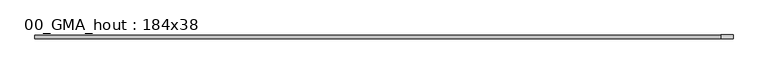
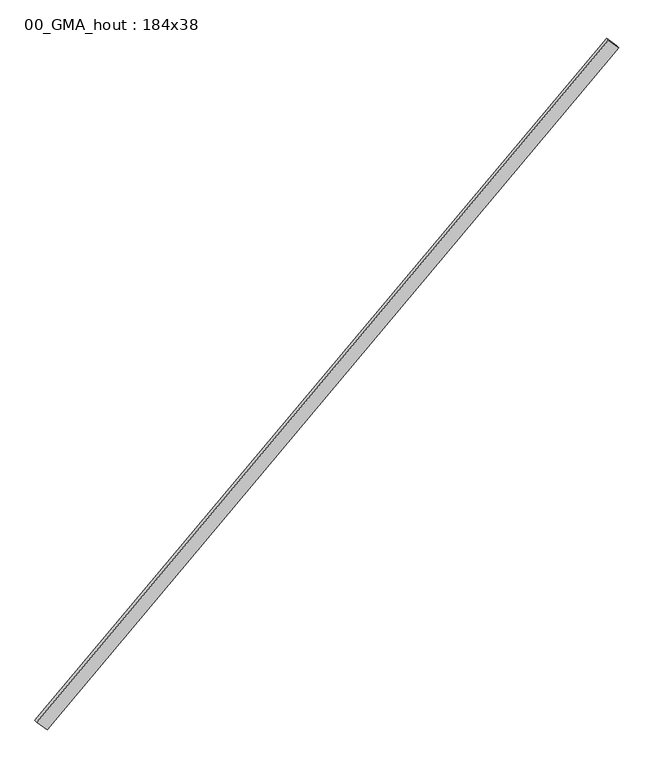
"""IFC4 building model written with IfcOpenShell, lengths in millimetres: proxy geometry, 00_GMA_hout : 184x38."""

import ifcopenshell
import ifcopenshell.guid

model = None  # the IFC model being written
_history = None  # IfcOwnerHistory: only IFC2X3 demands one
_inside = {}  # id of a spatial element -> (the spatial element, [elements in it])
_under = {}  # id of a project, library or spatial element -> (it, [spatial elements below it])
_declared = {}  # id of a project -> (the project, [libraries it declares])
_typed = {}  # id of a type object -> (the type object, [elements of that type])
_made_of = {}  # id of a material, layer set ... -> (it, [elements and type objects made of it])


def new_model(schema):
    """Start an empty IFC model of exactly this schema.

    Asked for "IFC4X3", IfcOpenShell would pick the latest addendum, in which some entities
    have other attributes; the version numbers below select the first issue.
    IFC2X3 requires an IfcOwnerHistory on every rooted entity: one is made here for all.
    """
    global model, _history
    if schema == "IFC4X3":
        model = ifcopenshell.file(schema_version=(4, 3, 0, 0))
    else:
        model = ifcopenshell.file(schema=schema)
    _inside.clear()
    _under.clear()
    _declared.clear()
    _typed.clear()
    _made_of.clear()
    _history = None
    if model.schema == "IFC2X3":
        org = make("IfcOrganization", Name="unknown")
        user = make(
            "IfcPersonAndOrganization",
            ThePerson=make("IfcPerson", FamilyName="unknown"),
            TheOrganization=org,
        )
        app = make(
            "IfcApplication",
            ApplicationDeveloper=org,
            Version="unknown",
            ApplicationFullName="unknown",
            ApplicationIdentifier="unknown",
        )
        _history = make(
            "IfcOwnerHistory",
            OwningUser=user,
            OwningApplication=app,
            ChangeAction="ADDED",
            CreationDate=0,
        )
    return model


def make(cls, **values):
    """One entity of the class cls with the attributes given. An attribute that is None is left unset."""
    return model.create_entity(
        cls, **{name: value for name, value in values.items() if value is not None}
    )


def rooted(cls, **values):
    """An entity with a GlobalId (a new one), such as an element, a storey or a relation."""
    return make(cls, GlobalId=ifcopenshell.guid.new(), OwnerHistory=_history, **values)


def si_unit(unit_type, name, prefix=None):
    """IfcSIUnit, for example si_unit("LENGTHUNIT", "METRE", prefix="MILLI")."""
    return make("IfcSIUnit", UnitType=unit_type, Prefix=prefix, Name=name)


def assignment(units):
    """IfcUnitAssignment: the units of a project."""
    return None if units is None else make("IfcUnitAssignment", Units=units)


def point(xyz):
    """IfcCartesianPoint."""
    return None if xyz is None else make("IfcCartesianPoint", Coordinates=xyz)


def direction(xyz):
    """IfcDirection."""
    return None if xyz is None else make("IfcDirection", DirectionRatios=xyz)


def frame(location, z_axis=None, x_axis=None):
    """IfcAxis2Placement3D, a coordinate frame: its origin and axes. An axis left out is left unset."""
    return make(
        "IfcAxis2Placement3D",
        Location=point(location),
        Axis=direction(z_axis),
        RefDirection=direction(x_axis),
    )


def origin():
    """The frame at (0, 0, 0) with its axes left unset."""
    return frame((0.0, 0.0, 0.0))


def place(relative_to, where):
    """IfcLocalPlacement: puts the frame where relative to a parent placement (None: the world)."""
    return make(
        "IfcLocalPlacement", PlacementRelTo=relative_to, RelativePlacement=where
    )


def context(
    kind, dimensions, precision=None, world=None, true_north=None, identifier=None
):
    """IfcGeometricRepresentationContext, for example the 3D "Model" context."""
    return make(
        "IfcGeometricRepresentationContext",
        ContextIdentifier=identifier,
        ContextType=kind,
        CoordinateSpaceDimension=dimensions,
        Precision=precision,
        WorldCoordinateSystem=world,
        TrueNorth=true_north,
    )


def project(units=None, contexts=None):
    """IfcProject with its units and contexts."""
    return rooted(
        "IfcProject",
        Name="project",
        RepresentationContexts=contexts,
        UnitsInContext=assignment(units),
    )


def spatial(cls, under=None, at=None, **own):
    """A site, building, storey or space (cls), placed at a placement, below another one or the project."""
    s = rooted(cls, ObjectPlacement=at, **own)
    if under is not None:
        _under.setdefault(under.id(), (under, []))[1].append(s)
    return s


def polyline(points):
    """IfcPolyline through the points."""
    return make("IfcPolyline", Points=[point(p) for p in points])


def outline(outer, holes=None, kind="AREA"):
    """IfcArbitraryClosedProfileDef: a profile drawn as a closed curve; with holes, ...WithVoids."""
    if holes is None:
        return make("IfcArbitraryClosedProfileDef", ProfileType=kind, OuterCurve=outer)
    return make(
        "IfcArbitraryProfileDefWithVoids",
        ProfileType=kind,
        OuterCurve=outer,
        InnerCurves=holes,
    )


def extrude(swept, where, along, depth):
    """IfcExtrudedAreaSolid: the profile swept, set in the frame where, extruded along a direction by depth."""
    return make(
        "IfcExtrudedAreaSolid",
        SweptArea=swept,
        Position=where,
        ExtrudedDirection=direction(along),
        Depth=depth,
    )


def shape(context_of_items, identifier, shape_type, items):
    """IfcShapeRepresentation: the items that make up one representation, for example the "Body"."""
    return make(
        "IfcShapeRepresentation",
        ContextOfItems=context_of_items,
        RepresentationIdentifier=identifier,
        RepresentationType=shape_type,
        Items=items,
    )


def source(mapping_origin, context_of_items, identifier, shape_type, items):
    """IfcRepresentationMap: a shape defined once, which mapped items show again and again."""
    return make(
        "IfcRepresentationMap",
        MappingOrigin=mapping_origin,
        MappedRepresentation=shape(context_of_items, identifier, shape_type, items),
    )


def transform(
    local_origin,
    x_axis=None,
    y_axis=None,
    z_axis=None,
    scale=None,
    scale2=None,
    scale3=None,
    uniform=True,
):
    """IfcCartesianTransformationOperator3D, or its non-uniform kind. x_axis, y_axis, z_axis: its Axis1, 2, 3."""
    if uniform:
        return make(
            "IfcCartesianTransformationOperator3D",
            Axis1=direction(x_axis),
            Axis2=direction(y_axis),
            LocalOrigin=point(local_origin),
            Scale=scale,
            Axis3=direction(z_axis),
        )
    return make(
        "IfcCartesianTransformationOperator3DnonUniform",
        Axis1=direction(x_axis),
        Axis2=direction(y_axis),
        LocalOrigin=point(local_origin),
        Scale=scale,
        Axis3=direction(z_axis),
        Scale2=scale2,
        Scale3=scale3,
    )


def mapped(mapping_source, mapping_target):
    """IfcMappedItem: shows the shape of a source again, moved by a transform."""
    return make(
        "IfcMappedItem", MappingSource=mapping_source, MappingTarget=mapping_target
    )


def made_of(thing, what):
    """Note that an element or type object is made of a material, layer set ...; save() writes the relation."""
    if what is not None:
        _made_of.setdefault(what.id(), (what, []))[1].append(thing)
    return thing


def element(
    cls,
    number,
    at=None,
    inside=None,
    cuts=None,
    type_object=None,
    material=None,
    context=None,
    identifier="Body",
    shape_type=None,
    held_by="IfcProductDefinitionShape",
    body=None,
    shapes=None,
    **own,
):
    """One element of the class cls, such as IfcWall. Its Tag is "e" and its number.

    at: its placement. inside: the storey or other place that contains it. cuts: it is an
    opening in that element (IfcRelVoidsElement). A single representation is given by context,
    identifier, shape_type and body (its items); several are given by shapes. held_by: the class
    of the entity that holds the representations. save() writes the other relations.
    """
    e = rooted(cls, Tag="e%d" % number, ObjectPlacement=at, **own)
    if body is not None:
        shapes = [shape(context, identifier, shape_type, body)]
    if shapes is not None:
        e.Representation = make(held_by, Representations=shapes)
    if inside is not None:
        _inside.setdefault(inside.id(), (inside, []))[1].append(e)
    if cuts is not None:
        rooted(
            "IfcRelVoidsElement", RelatingBuildingElement=cuts, RelatedOpeningElement=e
        )
    if type_object is not None:
        _typed.setdefault(type_object.id(), (type_object, []))[1].append(e)
    return made_of(e, material)


def aggregate(whole, parts):
    """IfcRelAggregates: a whole, such as a stair, and the parts it consists of."""
    return rooted("IfcRelAggregates", RelatingObject=whole, RelatedObjects=parts)


def save(model, path):
    """Write the relations noted so far, then the file.

    IfcRelAggregates (storeys below a building ...), IfcRelContainedInSpatialStructure (elements
    in a storey), IfcRelDefinesByType, IfcRelAssociatesMaterial and IfcRelDeclares: one each for
    every whole, place, type object, material and project.
    """
    for whole, parts in _under.values():
        aggregate(whole, parts)
    for where, things in _inside.values():
        rooted(
            "IfcRelContainedInSpatialStructure",
            RelatedElements=things,
            RelatingStructure=where,
        )
    for kind, things in _typed.values():
        rooted("IfcRelDefinesByType", RelatedObjects=things, RelatingType=kind)
    for what, things in _made_of.values():
        rooted("IfcRelAssociatesMaterial", RelatedObjects=things, RelatingMaterial=what)
    for by, libraries in _declared.values():
        rooted("IfcRelDeclares", RelatingContext=by, RelatedDefinitions=libraries)
    model.write(path)


def proxy_00_gma_hout_184x38_5b4af7b9(model_context):
    return source(origin(), model_context, "Body", "SweptSolid", [
        extrude(outline(polyline([(-19.0, 0.0), (19.0, 0.0), (19.0, -9193.2589372), (-19.0, -9193.2589372), (-19.0, 0.0)])), frame((-2830.5340948, 19.0, -2828.5000071), z_axis=(-0.67357883778224, 0.0, 0.7391153829355245), x_axis=(0.0, 1.0, 0.0)), (0.0, 0.0, 1.0), 184.0),
    ])


if __name__ == "__main__":
    model = new_model("IFC4")
    model_context = context("Model", 3, world=origin())
    ifc_project = project(units=[si_unit("LENGTHUNIT", "METRE", prefix="MILLI")], contexts=[model_context])
    site = spatial("IfcSite", under=ifc_project)
    building = spatial("IfcBuilding", under=site)
    placement = place(None, origin())
    proxy_00_gma_hout_184x38_shape = proxy_00_gma_hout_184x38_5b4af7b9(model_context)
    element("IfcBuildingElementProxy", 1, Name="00_GMA_hout : 184x38", ObjectType="00_GMA_hout : 184x38", at=placement, inside=building, context=model_context, shape_type="MappedRepresentation", body=[
        mapped(proxy_00_gma_hout_184x38_shape, transform((0.0, 0.0, 0.0), x_axis=(1.0, 0.0, 0.0), y_axis=(0.0, 1.0, 0.0), z_axis=(0.0, 0.0, 1.0))),
    ])
    save(model, "model.ifc")

# Revit data of these elements
# Type "00_GMA_hout : 184x38"
#   lengte [instance default] = 1198.641 mm
#   h = 38 mm
#   b = 184 mm
#   materiaal = 00_hout_vuren_generiek
#   PositionProfile [instance default] = 00_GMP_rectangle : TopLeft
#   Default Elevation = 0
# Element 1 (IfcBuildingElementProxy, "00_GMA_hout : 184x38")
#   lengte = 9193.259 mm
#   PositionProfile = 00_GMP_rectangle : TopRight
#   Materials on its faces: "00_hout_vuren_generiek"
# Materials
#   "00_hout_vuren_generiek": class "Wood", colour RGB 255 128 0, transparency 0, Manufacturer = "RevitGG", URL = "www.revitgg.nl", Description = "Hout, vuren, generiek", Cost = 0
